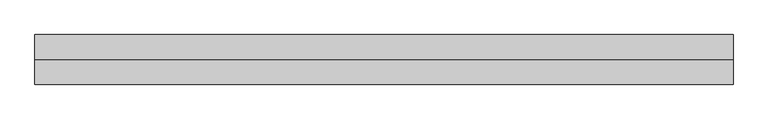
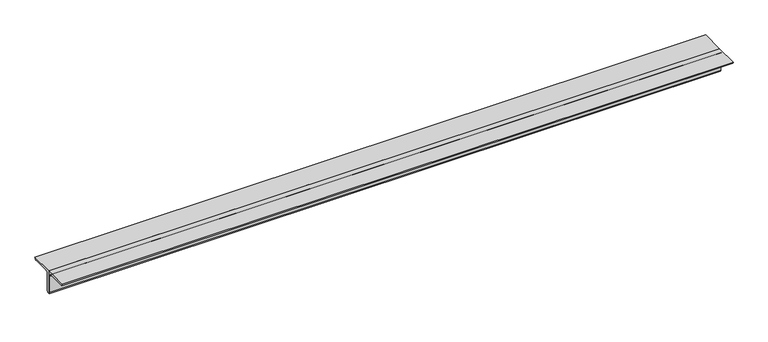
"""IFC4 building model written with IfcOpenShell, lengths in millimetres: member geometry, 0123_Steel Framing_2Ls-KSD3502 : H_SB_AR_S03_2Ls-130x130x12_HBR4."""

from ifc_helpers import new_model, si_unit, point, frame, frame_2d, origin, place, context, project, spatial, polyline, circle_curve, trimmed, segment, composite_curve, outline, extrude, source, transform, mapped, element, save


def member_a3ffd635(model_context):
    return source(origin(), model_context, "Body", "SweptSolid", [
        extrude(outline(composite_curve([segment(polyline([(0.0, 36.4), (130.0, 36.4)]), True, "CONTINUOUS"), segment(trimmed(circle_curve(frame_2d((118.0, 36.4)), 12.0), [point((130.0, 36.4))], [point((118.0, 24.4))], False, "CARTESIAN"), True, "CONTINUOUS"), segment(polyline([(118.0, 24.4), (24.0, 24.4)]), True, "CONTINUOUS"), segment(trimmed(circle_curve(frame_2d((24.0, 12.4)), 12.0), [point((24.0, 24.4))], [point((12.0, 12.4))], True, "CARTESIAN"), True, "CONTINUOUS"), segment(polyline([(12.0, 12.4), (12.0, -81.6)]), True, "CONTINUOUS"), segment(trimmed(circle_curve(frame_2d((0.0, -81.6)), 12.0), [point((12.0, -81.6))], [point((0.0, -93.6))], False, "CARTESIAN"), True, "CONTINUOUS"), segment(polyline([(0.0, -93.6), (0.0, 36.4)]), True, "CONTINUOUS")], self_intersect=False)), frame((-1939.8624184, 0.0, 0.0), z_axis=(1.0, 0.0, 0.0), x_axis=(0.0, 1.0, 0.0)), (0.0, 0.0, 1.0), 3660.0954461),
        extrude(outline(composite_curve([segment(polyline([(0.0, 36.4), (0.0, -93.6)]), True, "CONTINUOUS"), segment(trimmed(circle_curve(frame_2d((0.0, -81.6)), 12.0), [point((0.0, -93.6))], [point((-12.0, -81.6))], False, "CARTESIAN"), True, "CONTINUOUS"), segment(polyline([(-12.0, -81.6), (-12.0, 12.4)]), True, "CONTINUOUS"), segment(trimmed(circle_curve(frame_2d((-24.0, 12.4)), 12.0), [point((-12.0, 12.4))], [point((-24.0, 24.4))], True, "CARTESIAN"), True, "CONTINUOUS"), segment(polyline([(-24.0, 24.4), (-118.0, 24.4)]), True, "CONTINUOUS"), segment(trimmed(circle_curve(frame_2d((-118.0, 36.4)), 12.0), [point((-118.0, 24.4))], [point((-130.0, 36.4))], False, "CARTESIAN"), True, "CONTINUOUS"), segment(polyline([(-130.0, 36.4), (0.0, 36.4)]), True, "CONTINUOUS")], self_intersect=False)), frame((-1939.8624184, 0.0, 0.0), z_axis=(1.0, 0.0, 0.0), x_axis=(0.0, 1.0, 0.0)), (0.0, 0.0, 1.0), 3660.0954461),
    ])


if __name__ == "__main__":
    model = new_model("IFC4")
    model_context = context("Model", 3, world=origin())
    ifc_project = project(units=[si_unit("LENGTHUNIT", "METRE", prefix="MILLI")], contexts=[model_context])
    site = spatial("IfcSite", under=ifc_project)
    building = spatial("IfcBuilding", under=site)
    placement = place(None, origin())
    member_shape = member_a3ffd635(model_context)
    element("IfcMember", 1, ObjectType="0123_Steel Framing_2Ls-KSD3502 : H_SB_AR_S03_2Ls-130x130x12_HBR4", at=placement, inside=building, context=model_context, shape_type="MappedRepresentation", body=[
        mapped(member_shape, transform((0.0, 0.0, 0.0), x_axis=(1.0, 0.0, 0.0), y_axis=(0.0, 1.0, 0.0), z_axis=(0.0, 0.0, 1.0))),
    ])
    save(model, "model.ifc")

# Revit data of these elements
# Type "0123_Steel Framing_2Ls-KSD3502 : H_SB_AR_S03_2Ls-130x130x12_HBR4"
#   Type Mark = "HBR4"
#   Assembly Code = "B10"
#   Legs = "SLBB"
#   W = 8.97
#   Perimeter = 1.04 m²/m
#   Nominal Weight = 46.80 kgf/m
#   Length [instance default] = 1000 mm
#   Space = 0 mm
#   b = 130 mm
#   d = 130 mm
#   t = 12 mm
#   y = 36.4 mm
#   A = 0.005952 m²
#   Structural Material [instance default] = Steel ASTM A36
# Element 1 (IfcMember, "0123_Steel Framing_2Ls-KSD3502 : H_SB_AR_S03_2Ls-130x130x12_HBR4")
#   Materials on its faces: "Steel ASTM A36"
# Materials
#   "Steel ASTM A36": class "Metal", colour RGB 199 199 199, transparency 0, Description = "Structural steel, ASTM A36 Grade B, mill finish", Cost = 0
